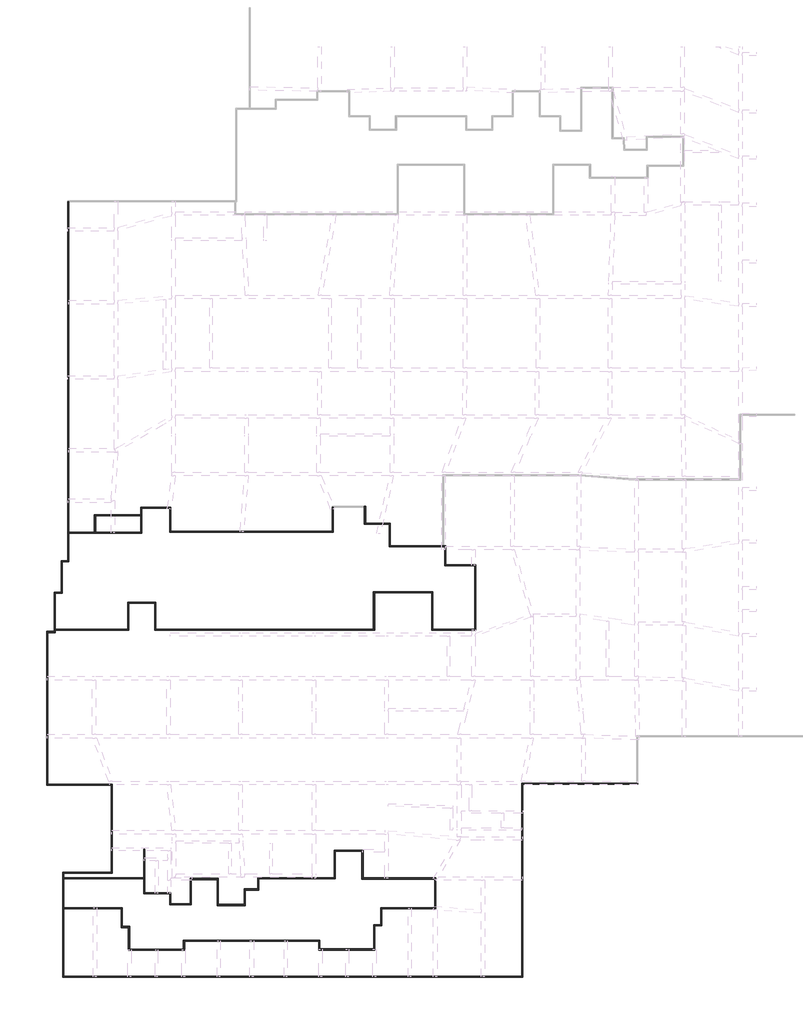
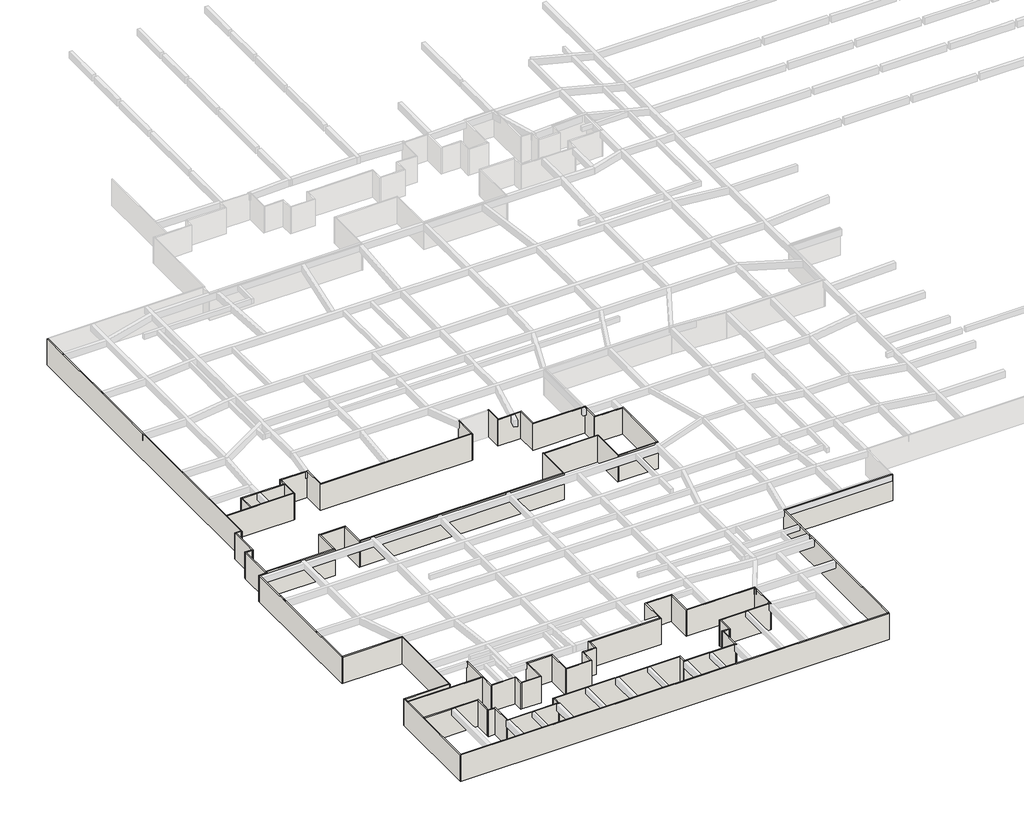
# One storey, part 1 of 16: 69 walls.
# Revit data of these elements (continued)
# Room, not placed, phase "新构造", upper offset 0 mm, lower offset 0 mm (continued)
#   Name = "客餐厅"
# Room, not placed, phase "新构造", upper offset 0 mm, lower offset 0 mm
#   Number = "2"
#   Name = "阳台"
# Room, not placed, phase "新构造", upper offset 0 mm, lower offset 0 mm
#   Number = "3"
#   Name = "次卧"
# Room, not placed, phase "新构造", upper offset 0 mm, lower offset 0 mm
#   Number = "4"
#   Name = "厨房"
# Room, not placed, phase "新构造", upper offset 0 mm, lower offset 0 mm
#   Number = "5"
#   Name = "卫生间"
# Room, not placed, phase "新构造", upper offset 0 mm, lower offset 0 mm
#   Number = "6"
#   Name = "次卧"
# Room, not placed, phase "新构造", upper offset 0 mm, lower offset 0 mm
#   Number = "7"
#   Name = "主卧"
# Area, not placed, upper offset 0 mm, lower offset 0 mm
#   Number = "60"
#   Name = "fire_compart"
# Area, not placed, upper offset 0 mm, lower offset 0 mm
#   Number = "23"
#   Name = "main_building"
# Area, not placed, upper offset 0 mm, lower offset 0 mm
#   Number = "36"
#   Name = "main_building"
# Area, not placed, upper offset 0 mm, lower offset 0 mm
#   Number = "37"
#   Name = "main_building"
# Area, not placed, upper offset 0 mm, lower offset 0 mm
#   Number = "38"
#   Name = "main_building"
# Area, not placed, upper offset 0 mm, lower offset 0 mm
#   Number = "39"
#   Name = "main_building"
# Area, not placed, upper offset 0 mm, lower offset 0 mm
#   Number = "40"
#   Name = "main_building"
# Area, not placed, upper offset 0 mm, lower offset 0 mm
#   Number = "64"
#   Name = "fire_compart"
# Area, not placed, upper offset 0 mm, lower offset 0 mm
#   Number = "61"
#   Name = "fire_compart"
# Area, not placed, upper offset 0 mm, lower offset 0 mm
#   Number = "65"
#   Name = "main_building"
# Area, not placed, upper offset 0 mm, lower offset 0 mm
#   Number = "62"
#   Name = "fire_compart"
# Area, not placed, upper offset 0 mm, lower offset 0 mm
#   Number = "63"
#   Name = "fire_compart"
# Area, not placed, upper offset 0 mm, lower offset 0 mm
#   Number = "66"
#   Name = "main_building"
# Area at (112709.366, 185693.512) mm, upper offset 0 mm, lower offset 0 mm
#   Number = "83"
#   Name = "fire_compart"
# Area at (111192.816, 204677.938) mm, upper offset 0 mm, lower offset 0 mm
#   Number = "84"
#   Name = "main_building"
# Area, not placed, upper offset 0 mm, lower offset 0 mm
#   Number = "7"
#   Name = "fire_compart_5"
# Area, not placed, upper offset 0 mm, lower offset 0 mm
#   Number = "67"
#   Name = "fire_compart"
# Area, not placed, upper offset 0 mm, lower offset 0 mm
#   Number = "68"
#   Name = "fire_compart"
# Area, not placed, upper offset 0 mm, lower offset 0 mm
#   Number = "1"
#   Name = "面积"
# Area, not placed, upper offset 0 mm, lower offset 0 mm
#   Number = "2"
#   Name = "防火区域1"
# Area, not placed, upper offset 0 mm, lower offset 0 mm
#   Number = "25"
#   Name = "fire_compart"
# Area, not placed, upper offset 0 mm, lower offset 0 mm
#   Number = "26"
#   Name = "fire_compart"
# Area, not placed, upper offset 0 mm, lower offset 0 mm
#   Number = "27"
#   Name = "fire_compart"
# Area, not placed, upper offset 0 mm, lower offset 0 mm
#   Number = "69"
#   Name = "fire_compart"
# Area at (172355.776, 108986.581) mm, upper offset 0 mm, lower offset 0 mm
#   Number = "95"
#   Name = "fire_compart"
# Area at (208379.065, 104280.021) mm, upper offset 0 mm, lower offset 0 mm
#   Number = "96"
#   Name = "main_building"
# Area at (168747.058, 122832.523) mm, upper offset 0 mm, lower offset 0 mm
#   Number = "97"
#   Name = "main_building"
# Area at (178870.842, 183143.05) mm, upper offset 0 mm, lower offset 0 mm
#   Number = "85"
#   Name = "fire_compart"
# Area at (180387.392, 205600.443) mm, upper offset 0 mm, lower offset 0 mm
#   Number = "86"
#   Name = "main_building"
# Area at (159883.994, 201201.94) mm, upper offset 0 mm, lower offset 0 mm
#   Number = "87"
#   Name = "main_building"
# Room, not placed, phase "新构造", upper offset 0 mm, lower offset 0 mm
#   Number = "8"
#   Name = "客餐厅"
# Area, not placed, upper offset 0 mm, lower offset 0 mm
#   Number = "70"
#   Name = "main_building"
# Area, not placed, upper offset 0 mm, lower offset 0 mm
#   Number = "8"
#   Name = "fire_compart_6"
# Area, not placed, upper offset 0 mm, lower offset 0 mm
#   Number = "3"
#   Name = "fire_compart_1"
# Area, not placed, upper offset 0 mm, lower offset 0 mm
#   Number = "71"
#   Name = "fire_compart"
# Room, not placed, phase "新构造", upper offset 0 mm, lower offset 0 mm
#   Number = "11"
#   Name = "房间"
# Room, not placed, phase "新构造", upper offset 0 mm, lower offset 0 mm
#   Number = "12"
#   Name = "房间"
# Room, not placed, phase "新构造", upper offset 0 mm, lower offset 0 mm
#   Number = "13"
#   Name = "房间"
# Room, not placed, phase "新构造", upper offset 0 mm, lower offset 0 mm
#   Number = "14"
#   Name = "房间"
# Area, not placed, upper offset 0 mm, lower offset 0 mm
#   Number = "72"
#   Name = "main_building"
# Room, not placed, phase "新构造", upper offset 0 mm, lower offset 0 mm
#   Number = "15"
#   Name = "房间"
# Area at (101333.607, 131847.351) mm, upper offset 0 mm, lower offset 0 mm
#   Number = "88"
#   Name = "fire_compart"
# Room, not placed, phase "新构造", upper offset 0 mm, lower offset 0 mm
#   Number = "16"
#   Name = "房间"
# Area, not placed, upper offset 0 mm, lower offset 0 mm
#   Number = "28"
#   Name = "面积"
# Area, not placed, upper offset 0 mm, lower offset 0 mm
#   Number = "73"
#   Name = "fire_compart"
# Room, not placed, phase "新构造", upper offset 0 mm, lower offset 0 mm
#   Number = "17"
#   Name = "房间"
# Area, not placed, upper offset 0 mm, lower offset 0 mm
#   Number = "30"
#   Name = "main_building"
# Area at (87985.305, 86907.237) mm, upper offset 0 mm, lower offset 0 mm
#   Number = "92"
#   Name = "fire_compart"
# Area at (89501.855, 66680.046) mm, upper offset 0 mm, lower offset 0 mm
#   Number = "93"
#   Name = "main_building"
# Area at (101702.313, 151799.58) mm, upper offset 0 mm, lower offset 0 mm
#   Number = "89"
#   Name = "main_building"
# Area, not placed, upper offset 0 mm, lower offset 0 mm
#   Number = "75"
#   Name = "main_building"
# Area at (133088.348, 159635.722) mm, upper offset 0 mm, lower offset 0 mm
#   Number = "90"
#   Name = "fire_compart"
# Area, not placed, upper offset 0 mm, lower offset 0 mm
#   Number = "76"
#   Name = "main_building"
# Area, not placed, upper offset 0 mm, lower offset 0 mm
#   Number = "4"
#   Name = "fire_compart_2"
# Area at (77235.846, 104980.22) mm, upper offset 0 mm, lower offset 0 mm
#   Number = "94"
#   Name = "main_building"
# Area, not placed, upper offset 0 mm, lower offset 0 mm
#   Number = "77"
#   Name = "main_building"
# Area, not placed, upper offset 0 mm, lower offset 0 mm
#   Number = "78"
#   Name = "main_building"
# Area, not placed, upper offset 0 mm, lower offset 0 mm
#   Number = "79"
#   Name = "main_building"
# Area, not placed, upper offset 0 mm, lower offset 0 mm
#   Number = "29"
#   Name = "main_building"
